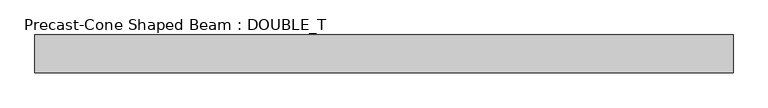
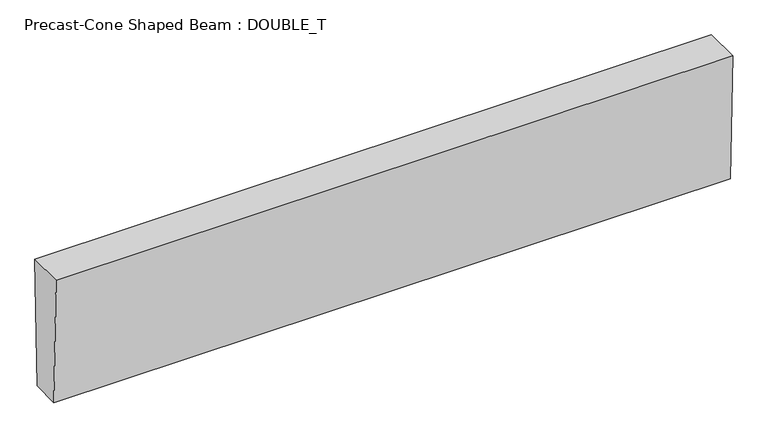
"""IFC4 building model written with IfcOpenShell, lengths in millimetres: beam geometry, Precast-Cone Shaped Beam : DOUBLE_T."""

from ifc_helpers import new_model, si_unit, frame, origin, place, context, project, spatial, polyline, outline, extrude, source, transform, mapped, element, save


def precast_cone_shaped_beam_double_t_7663fcfe(model_context):
    return source(origin(), model_context, "Body", "SweptSolid", [
        extrude(outline(polyline([(-50.8, -228.6), (-63.5, 228.6), (63.5, 228.6), (50.8, -228.6), (-50.8, -228.6)])), frame((-1119.0263686, 0.0, 0.0), z_axis=(1.0, 0.0, 0.0), x_axis=(0.0, 1.0, 0.0)), (0.0, 0.0, 1.0), 2347.5902372),
    ])


if __name__ == "__main__":
    model = new_model("IFC4")
    model_context = context("Model", 3, world=origin())
    ifc_project = project(units=[si_unit("LENGTHUNIT", "METRE", prefix="MILLI")], contexts=[model_context])
    site = spatial("IfcSite", under=ifc_project)
    building = spatial("IfcBuilding", under=site)
    placement = place(None, origin())
    precast_cone_shaped_beam_double_t_shape = precast_cone_shaped_beam_double_t_7663fcfe(model_context)
    element("IfcBeam", 1, ObjectType="Precast-Cone Shaped Beam : DOUBLE_T", at=placement, inside=building, context=model_context, shape_type="MappedRepresentation", body=[
        mapped(precast_cone_shaped_beam_double_t_shape, transform((0.0, 0.0, 0.0), x_axis=(1.0, 0.0, 0.0), y_axis=(0.0, 1.0, 0.0), z_axis=(0.0, 0.0, 1.0))),
    ])
    save(model, "model.ifc")

# Revit data of these elements
# Type "Precast-Cone Shaped Beam : DOUBLE_T"
#   Top Width = 0' - 5"
#   Tie Rod Weight [instance default] = 30
#   Tie Rod W [instance default] = 0.0660938 kip
#   Single Rebar Weight [instance default] = 50
#   Single Rebar W [instance default] = 0.110156 kip
#   Rebar Grids Weight [instance default] = 100
#   Rebar Grids W [instance default] = 0.220313 kip
#   Depth = 1' - 6"
#   Bottom Width = 0' - 4"
#   Length [instance default] = 5' - 0"
#   Structural Material [instance default] = Concrete, Precast
#   Assembly Code = ""
# Element 1 (IfcBeam, "Precast-Cone Shaped Beam : DOUBLE_T")
#   Length = 7' - 4.11231"
#   Structural Material = Concrete - Precast Concrete - Normal Weight Concrete - 5 ksi
#   Materials on its faces: "Concrete - Precast Concrete - Normal Weight Concrete - 5 ksi"
# Materials
#   "Concrete, Precast": class "Concrete", colour RGB 198 187 187, transparency 0, Description = "Precast concrete", Cost = 0
#   "Concrete - Precast Concrete - Normal Weight Concrete - 5 ksi": class "Concrete", colour RGB 198 187 187, transparency 0, Cost = 0
